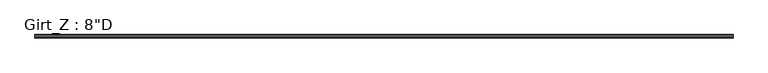
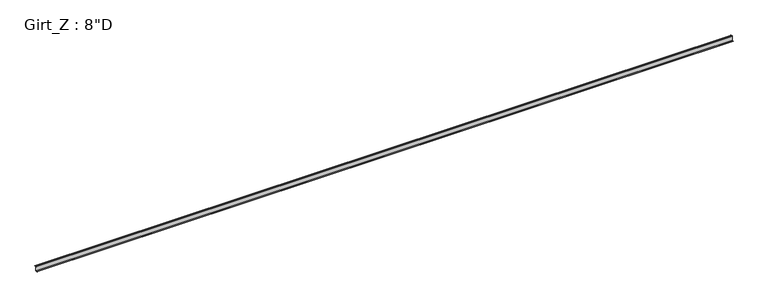
"""IFC4 building model written with IfcOpenShell, lengths in millimetres: beam geometry."""

from ifc_helpers import new_model, si_unit, point, frame, frame_2d, origin, place, context, project, spatial, polyline, circle_curve, trimmed, segment, composite_curve, outline, extrude, source, transform, mapped, element, save


def beam_e2549a39(model_context):
    return source(origin(), model_context, "Body", "SweptSolid", [
        extrude(outline(composite_curve([segment(polyline([(63.5, 101.6), (75.745104, 87.0068534), (73.6169367, 85.221109), (62.204539, 98.821875), (3.3005807, 98.821875)]), True, "CONTINUOUS"), segment(trimmed(circle_curve(frame_2d((3.3741066, 96.8381931)), 1.9850441), [point((3.3005807, 98.821875))], [point((1.3890625, 96.8381931))], True, "CARTESIAN"), True, "CONTINUOUS"), segment(polyline([(1.3890625, 96.8381931), (1.3890625, -96.8375)]), True, "CONTINUOUS"), segment(trimmed(circle_curve(frame_2d((-3.3734375, -96.8375)), 4.7625), [point((1.3890625, -96.8375))], [point((-3.3734375, -101.6))], False, "CARTESIAN"), True, "CONTINUOUS"), segment(polyline([(-3.3734375, -101.6), (-63.5, -101.6), (-75.745104, -87.0068534), (-73.6169367, -85.221109), (-62.204539, -98.821875), (-3.2694106, -98.821875)]), True, "CONTINUOUS"), segment(trimmed(circle_curve(frame_2d((-3.3748024, -96.8389339)), 1.9857399), [point((-3.2694106, -98.821875))], [point((-1.3890625, -96.8389339))], True, "CARTESIAN"), True, "CONTINUOUS"), segment(polyline([(-1.3890625, -96.8389339), (-1.3890625, 96.8375)]), True, "CONTINUOUS"), segment(trimmed(circle_curve(frame_2d((3.3734375, 96.8375)), 4.7625), [point((-1.3890625, 96.8375))], [point((3.3734375, 101.6))], False, "CARTESIAN"), True, "CONTINUOUS"), segment(polyline([(3.3734375, 101.6), (63.5, 101.6)]), True, "CONTINUOUS")], self_intersect=False)), frame((-15595.6, 0.0, 0.0), z_axis=(1.0, 0.0, 0.0), x_axis=(0.0, 1.0, 0.0)), (0.0, 0.0, 1.0), 29895.5150467),
    ])


if __name__ == "__main__":
    model = new_model("IFC4")
    model_context = context("Model", 3, world=origin())
    ifc_project = project(units=[si_unit("LENGTHUNIT", "METRE", prefix="MILLI")], contexts=[model_context])
    site = spatial("IfcSite", under=ifc_project)
    building = spatial("IfcBuilding", under=site)
    placement = place(None, origin())
    beam_shape = beam_e2549a39(model_context)
    element("IfcBeam", 1, ObjectType="Girt_Z : 8\"D", at=placement, inside=building, context=model_context, shape_type="MappedRepresentation", body=[
        mapped(beam_shape, transform((0.0, 0.0, 0.0), x_axis=(1.0, 0.0, 0.0), y_axis=(0.0, 1.0, 0.0), z_axis=(0.0, 0.0, 1.0))),
    ])
    save(model, "model.ifc")

# Revit data of these elements
# Type "Girt_Z : 8\"D"
#   Web_Thickness = 0' - 0 7/64"
#   Length [instance default] = 10' - 0"
#   Leg_1 = 0' - 2 1/2"
#   Height = 0' - 8"
#   Structural Material [instance default] = none
# Element 1 (IfcBeam, "Girt_Z : 8\"D")
#   Structural Material = Steel
#   Materials on its faces: "Steel"
# Materials
#   "Steel": class "Metal", colour RGB 118 118 114, transparency 0, Description = "Steel, mill finish", Cost = 0
